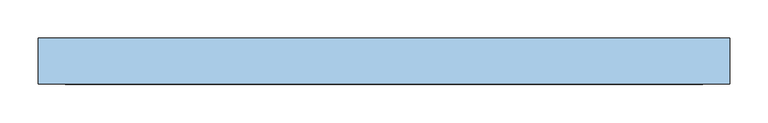
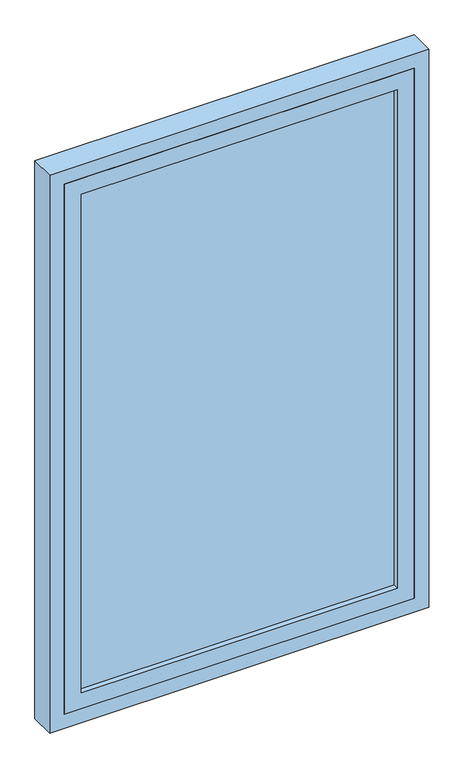
"""IFC4 building model written with IfcOpenShell, lengths in millimetres: window geometry, Janela fixa - 1 Painel : Janela fixa - 1 Painel."""

from ifc_helpers import new_model, si_unit, frame, origin, place, context, project, spatial, polyline, outline, extrude, source, transform, mapped, element, save


def window_e4a1cf9c(model_context):
    return source(origin(), model_context, "Body", "SweptSolid", [
        extrude(outline(polyline([(375.0, -73.0), (375.0, -87.0), (-375.0, -87.0), (-375.0, -73.0), (375.0, -73.0)])), frame((0.0, 0.0, 725.0), z_axis=(0.0, 0.0, 1.0), x_axis=(1.0, 0.0, 0.0)), (0.0, 0.0, 1.0), 1250.0),
        extrude(outline(polyline([(685.0, -415.0), (685.0, 415.0), (2015.0, 415.0), (2015.0, -415.0), (685.0, -415.0)]), holes=[polyline([(1975.0, -375.0), (1975.0, 375.0), (725.0, 375.0), (725.0, -375.0), (1975.0, -375.0)])]), frame((0.0, -100.0, 0.0), z_axis=(0.0, 1.0, 0.0), x_axis=(0.0, 0.0, 1.0)), (0.0, 0.0, 1.0), 40.0),
        extrude(outline(polyline([(650.0, -450.0), (650.0, 450.0), (2050.0, 450.0), (2050.0, -450.0), (650.0, -450.0)]), holes=[polyline([(2015.0, -415.0), (2015.0, 415.0), (685.0, 415.0), (685.0, -415.0), (2015.0, -415.0)])]), frame((0.0, -100.0, 0.0), z_axis=(0.0, 1.0, 0.0), x_axis=(0.0, 0.0, 1.0)), (0.0, 0.0, 1.0), 60.0),
    ])


if __name__ == "__main__":
    model = new_model("IFC4")
    model_context = context("Model", 3, world=origin())
    ifc_project = project(units=[si_unit("LENGTHUNIT", "METRE", prefix="MILLI")], contexts=[model_context])
    site = spatial("IfcSite", under=ifc_project)
    building = spatial("IfcBuilding", under=site)
    placement = place(None, origin())
    window_shape = window_e4a1cf9c(model_context)
    element("IfcWindow", 1, ObjectType="Janela fixa - 1 Painel : Janela fixa - 1 Painel", at=placement, inside=building, context=model_context, shape_type="MappedRepresentation", body=[
        mapped(window_shape, transform((0.0, 0.0, 0.0), x_axis=(1.0, 0.0, 0.0), y_axis=(0.0, 1.0, 0.0), z_axis=(0.0, 0.0, 1.0))),
    ])
    save(model, "model.ifc")

# Revit data of these elements
# Type "Janela fixa - 1 Painel : Janela fixa - 1 Painel"
#   Type Mark = "19"
#   Construction Type Id = "SGL"
#   Analytic Construction = "Janelas grandes envidraçadas únicas"
#   Visual Light Transmittance = 0.9
#   Solar Heat Gain Coefficient = 0.86
#   Rough Width = 900 mm
#   Rough Height = 1400 mm
#   Largura da moldura do painel = 40 mm
#   Espessura da moldura do painel = 40 mm
#   Height = 1400 mm
#   Heat Transfer Coefficient (U) = 5.5617 W/(m²·K)
#   Largura da estrutura = 35 mm
#   Espessura da moldura = 60 mm
#   Altura-padrão do peitoril = 650 mm
#   Width = 900 mm
#   Vidro = none
#   Material da moldura = none
#   Wall Closure = (empty or 0)
# Element 1 (IfcWindow, "Janela fixa - 1 Painel : Janela fixa - 1 Painel")
#   Materials on its faces: "Vidro"
# Materials
#   "Vidro": class "Vidro", colour RGB 0 128 192, transparency 0.9, Description = "Vidro de sílica", Cost = 0
